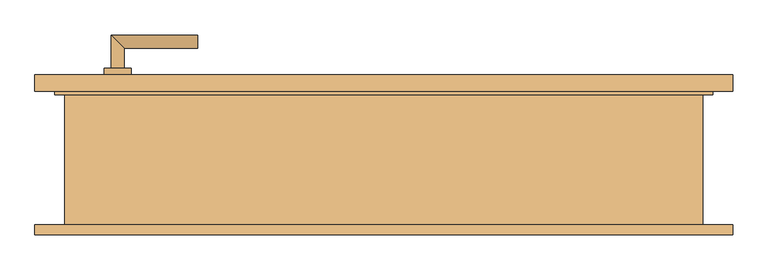
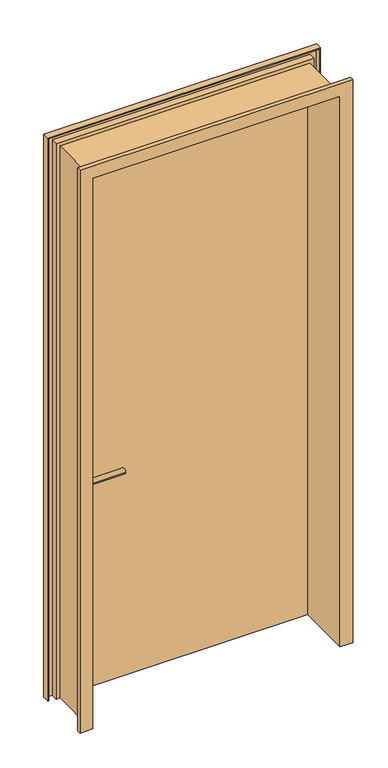
"""IFC4 building model written with IfcOpenShell, lengths in millimetres: door geometry, Drehflügel 1-flg - Variabel : Drehflügel 1-flg - Variabel."""

from ifc_helpers import new_model, si_unit, point, frame, frame_2d, origin, origin_with_axes, place, context, project, spatial, polyline, circle_curve, ellipse_curve, trimmed, segment, composite_curve, outline, extrude, faceted_brep, source, transform, mapped, element, save
from ifc_brep_helpers import plane_surface, cylinder_surface, advanced_brep


def door_75bb7ed5(model_context):
    return source(origin(), model_context, "Body", "SolidModel", [
        advanced_brep(
        [(-410.0, 89.4346141, 900.0), (-390.0, 89.4346141, 900.0), (-410.0, 19.4346141, 900.0), (-390.0, 39.4346141, 900.0), (-280.0, 19.4346141, 900.0), (-280.0, 39.4346141, 900.0)],
        [
            (0, 1, circle_curve(frame((-400.0, 89.4346141, 900.0), z_axis=(0.0, 1.0, 0.0), x_axis=(1.0, 0.0, 0.0)), 10.0)),
            (1, 0, circle_curve(frame((-400.0, 89.4346141, 900.0), z_axis=(0.0, 1.0, 0.0), x_axis=(1.0, 0.0, 0.0)), 10.0)),
            (0, 2),
            (2, 3, ellipse_curve(frame((-400.0, 29.4346141, 900.0), z_axis=(-0.7071067811865385, 0.7071067811865565, 0.0), x_axis=(0.7071067811865563, 0.7071067811865386, 0.0)), 14.1421356, 10.0)),
            (3, 1),
            (3, 2, ellipse_curve(frame((-400.0, 29.4346141, 900.0), z_axis=(-0.7071067811865385, 0.7071067811865565, 0.0), x_axis=(0.7071067811865563, 0.7071067811865386, 0.0)), 14.1421356, 10.0)),
            (4, 5, circle_curve(frame((-280.0, 29.4346141, 900.0), z_axis=(1.0, 0.0, 0.0), x_axis=(0.0, 1.0, 0.0)), 10.0)),
            (5, 4, circle_curve(frame((-280.0, 29.4346141, 900.0), z_axis=(1.0, 0.0, 0.0), x_axis=(0.0, 1.0, 0.0)), 10.0)),
            (2, 4),
            (5, 3),
        ],
        [
            plane_surface(frame((-400.0, 89.4346141, -387.7526403), z_axis=(0.0, 1.0, 0.0), x_axis=(0.0, 0.0, 1.0))),
            cylinder_surface(frame((-400.0, 89.4346141, 900.0), z_axis=(0.0, 1.0, 0.0), x_axis=(1.0, 0.0, 0.0)), 10.0),
            plane_surface(frame((-280.0, 29.4346141, -387.7526403), z_axis=(1.0, 0.0, 0.0), x_axis=(0.0, 0.0, 1.0))),
            cylinder_surface(frame((-400.0, 29.4346141, 900.0), z_axis=(-1.0, 0.0, 0.0), x_axis=(0.0, 1.0, 0.0)), 10.0),
        ],
        [
            (0, [[1, 2]]),
            (1, [[-1, 3, 4, 5]]),
            (1, [[-2, -5, 6, -3]]),
            (2, [[7, 8]]),
            (3, [[-4, 9, -8, 10]]),
            (3, [[-6, -10, -7, -9]]),
        ],
    ),
        advanced_brep(
        [(-390.0, 149.4346141, 900.0), (-410.0, 149.4346141, 900.0), (-390.0, 179.4346141, 900.0), (-410.0, 199.4346141, 900.0), (-280.0, 179.4346141, 900.0), (-280.0, 199.4346141, 900.0)],
        [
            (0, 1, circle_curve(frame((-400.0, 149.4346141, 900.0), z_axis=(0.0, -1.0, 0.0), x_axis=(-1.0, 0.0, 0.0)), 10.0)),
            (1, 0, circle_curve(frame((-400.0, 149.4346141, 900.0), z_axis=(0.0, -1.0, 0.0), x_axis=(-1.0, 0.0, 0.0)), 10.0)),
            (0, 2),
            (2, 3, ellipse_curve(frame((-400.0, 189.4346141, 900.0), z_axis=(-0.7071067811865475, -0.7071067811865475, 0.0), x_axis=(0.7071067811865474, -0.7071067811865476, 0.0)), 14.1421356, 10.0)),
            (3, 1),
            (3, 2, ellipse_curve(frame((-400.0, 189.4346141, 900.0), z_axis=(-0.7071067811865475, -0.7071067811865475, 0.0), x_axis=(0.7071067811865474, -0.7071067811865476, 0.0)), 14.1421356, 10.0)),
            (4, 5, circle_curve(frame((-280.0, 189.4346141, 900.0), z_axis=(1.0, 0.0, 0.0), x_axis=(0.0, 1.0, 0.0)), 10.0)),
            (5, 4, circle_curve(frame((-280.0, 189.4346141, 900.0), z_axis=(1.0, 0.0, 0.0), x_axis=(0.0, 1.0, 0.0)), 10.0)),
            (2, 4),
            (5, 3),
        ],
        [
            plane_surface(frame((-400.0, 149.4346141, -387.7526403), z_axis=(0.0, -1.0, 0.0), x_axis=(0.0, 0.0, 1.0))),
            cylinder_surface(frame((-400.0, 149.4346141, 900.0), z_axis=(0.0, -1.0, 0.0), x_axis=(-1.0, 0.0, 0.0)), 10.0),
            plane_surface(frame((-280.0, 189.4346141, -387.7526403), z_axis=(1.0, 0.0, 0.0), x_axis=(0.0, 0.0, 1.0))),
            cylinder_surface(frame((-400.0, 189.4346141, 900.0), z_axis=(-1.0, 0.0, 0.0), x_axis=(0.0, 1.0, 0.0)), 10.0),
        ],
        [
            (0, [[1, 2]]),
            (1, [[-1, 3, 4, 5]]),
            (1, [[-2, -5, 6, -3]]),
            (2, [[7, 8]]),
            (3, [[-4, 9, -8, 10]]),
            (3, [[-6, -10, -7, -9]]),
        ],
    ),
        extrude(outline(composite_curve([segment(trimmed(circle_curve(frame_2d((900.0, -400.0)), 20.0), [point((900.0, -420.0))], [point((900.0, -380.0))], False, "CARTESIAN"), True, "CONTINUOUS"), segment(trimmed(circle_curve(frame_2d((900.0, -400.0)), 20.0), [point((900.0, -380.0))], [point((900.0, -420.0))], False, "CARTESIAN"), True, "CONTINUOUS")], self_intersect=False)), frame((0.0, 79.4346141, 0.0), z_axis=(0.0, 1.0, 0.0), x_axis=(0.0, 0.0, 1.0)), (0.0, 0.0, 1.0), 10.0),
        extrude(outline(composite_curve([segment(trimmed(circle_curve(frame_2d((900.0, -400.0)), 20.0), [point((900.0, -420.0))], [point((900.0, -380.0))], False, "CARTESIAN"), True, "CONTINUOUS"), segment(trimmed(circle_curve(frame_2d((900.0, -400.0)), 20.0), [point((900.0, -380.0))], [point((900.0, -420.0))], False, "CARTESIAN"), True, "CONTINUOUS")], self_intersect=False)), frame((0.0, 139.4346141, 0.0), z_axis=(0.0, 1.0, 0.0), x_axis=(0.0, 0.0, 1.0)), (0.0, 0.0, 1.0), 10.0),
        extrude(outline(polyline([(490.0, 114.4346141), (-490.0, 114.4346141), (-490.0, 139.4346141), (490.0, 139.4346141), (490.0, 114.4346141)])), origin_with_axes(), (0.0, 0.0, 1.0), 2250.0),
        faceted_brep([(524.4603207, -100.5653859, 0.0), (475.0, -100.5653859, 0.0), (475.0, 114.4346141, 0.0), (490.0, 114.4346141, 0.0), (490.0, 139.4346141, 0.0), (524.4603207, 139.4346141, 0.0), (524.4603207, 114.4346141, 0.0), (519.4603207, 114.4346141, 0.0), (519.4603207, 134.4346141, 0.0), (495.0, 134.4346141, 0.0), (495.0, 109.4346141, 0.0), (480.0, 109.4346141, 0.0), (480.0, -95.5653859, 0.0), (519.4603207, -95.5653859, 0.0), (519.4603207, -85.5653859, 0.0), (524.4603207, -85.5653859, 0.0), (524.4603207, -100.5653859, 2284.4603207), (-524.4603207, -100.5653859, 2284.4603207), (-524.4603207, -100.5653859, 0.0), (-475.0, -100.5653859, 0.0), (-475.0, -100.5653859, 2235.0), (475.0, -100.5653859, 2235.0), (475.0, 114.4346141, 2235.0), (-475.0, 114.4346141, 2235.0), (-475.0, 114.4346141, 0.0), (-490.0, 114.4346141, 0.0), (-490.0, 114.4346141, 2250.0), (490.0, 114.4346141, 2250.0), (490.0, 139.4346141, 2250.0), (-490.0, 139.4346141, 2250.0), (-490.0, 139.4346141, 0.0), (-524.4603207, 139.4346141, 0.0), (-524.4603207, 139.4346141, 2284.4603207), (524.4603207, 139.4346141, 2284.4603207), (524.4603207, 114.4346141, 2284.4603207), (-524.4603207, 114.4346141, 2284.4603207), (-524.4603207, 114.4346141, 0.0), (-519.4603207, 114.4346141, 0.0), (-519.4603207, 114.4346141, 2279.4603207), (519.4603207, 114.4346141, 2279.4603207), (519.4603207, 134.4346141, 2279.4603207), (-519.4603207, 134.4346141, 2279.4603207), (-519.4603207, 134.4346141, 0.0), (-495.0, 134.4346141, 0.0), (-495.0, 134.4346141, 2255.0), (495.0, 134.4346141, 2255.0), (495.0, 109.4346141, 2255.0), (-495.0, 109.4346141, 2255.0), (-495.0, 109.4346141, 0.0), (-480.0, 109.4346141, 0.0), (-480.0, 109.4346141, 2240.0), (480.0, 109.4346141, 2240.0), (480.0, -95.5653859, 2240.0), (-480.0, -95.5653859, 2240.0), (-480.0, -95.5653859, 0.0), (-519.4603207, -95.5653859, 0.0), (-519.4603207, -95.5653859, 2279.4603207), (519.4603207, -95.5653859, 2279.4603207), (519.4603207, -85.5653859, 2279.4603207), (-519.4603207, -85.5653859, 2279.4603207), (-519.4603207, -85.5653859, 0.0), (-524.4603207, -85.5653859, 0.0), (-524.4603207, -85.5653859, 2284.4603207), (524.4603207, -85.5653859, 2284.4603207)], [[[0, 1, 2, 3, 4, 5, 6, 7, 8, 9, 10, 11, 12, 13, 14, 15]], [[1, 0, 16, 17, 18, 19, 20, 21]], [[2, 1, 21, 22]], [[3, 2, 22, 23, 24, 25, 26, 27]], [[4, 3, 27, 28]], [[5, 4, 28, 29, 30, 31, 32, 33]], [[6, 5, 33, 34]], [[7, 6, 34, 35, 36, 37, 38, 39]], [[8, 7, 39, 40]], [[9, 8, 40, 41, 42, 43, 44, 45]], [[10, 9, 45, 46]], [[11, 10, 46, 47, 48, 49, 50, 51]], [[12, 11, 51, 52]], [[13, 12, 52, 53, 54, 55, 56, 57]], [[14, 13, 57, 58]], [[15, 14, 58, 59, 60, 61, 62, 63]], [[0, 15, 63, 16]], [[17, 62, 61, 18]], [[18, 61, 60, 55, 54, 49, 48, 43, 42, 37, 36, 31, 30, 25, 24, 19]], [[23, 20, 19, 24]], [[29, 26, 25, 30]], [[35, 32, 31, 36]], [[41, 38, 37, 42]], [[47, 44, 43, 48]], [[53, 50, 49, 54]], [[59, 56, 55, 60]], [[22, 21, 20, 23]], [[28, 27, 26, 29]], [[34, 33, 32, 35]], [[40, 39, 38, 41]], [[46, 45, 44, 47]], [[52, 51, 50, 53]], [[58, 57, 56, 59]], [[16, 63, 62, 17]]]),
    ])


if __name__ == "__main__":
    model = new_model("IFC4")
    model_context = context("Model", 3, world=origin())
    ifc_project = project(units=[si_unit("LENGTHUNIT", "METRE", prefix="MILLI")], contexts=[model_context])
    site = spatial("IfcSite", under=ifc_project)
    building = spatial("IfcBuilding", under=site)
    placement = place(None, origin())
    door_shape = door_75bb7ed5(model_context)
    element("IfcDoor", 1, ObjectType="Drehflügel 1-flg - Variabel : Drehflügel 1-flg - Variabel", at=placement, inside=building, context=model_context, shape_type="MappedRepresentation", body=[
        mapped(door_shape, transform((0.0, 0.0, 0.0), x_axis=(1.0, 0.0, 0.0), y_axis=(0.0, 1.0, 0.0), z_axis=(0.0, 0.0, 1.0))),
    ])
    save(model, "model.ifc")

# Revit data of these elements
# Type "Drehflügel 1-flg - Variabel : Drehflügel 1-flg - Variabel"
#   Construction Type Id = "MDOOR"
#   Type Mark = "15"
#   Operation = "SingleSwingRight"
#   Keynote = "16.03"
#   Analytic Construction = "Metall"
#   Thermal Resistance (R) = 0.270117 (m²·K)/W
#   Heat Transfer Coefficient (U) = 3.7021 W/(m²·K)
#   Rough Width [instance default] = 1.000 m
#   Rough Height [instance default] = 2.360 m
#   Höhe Türgriff [instance default] = 0.900 m
#   Height [instance default] = 2.260 m
#   Fußbodenaufbau [instance default] = 0.100 m
#   Width [instance default] = 1.000 m
#   Sichtbarkeit Sturzlinien [instance default] = yes
#   Türgriff auswählen [instance default] = element 217699
#   Türgriff [instance default] = none
#   Türflügel [instance default] = none
#   Rahmen/Pfosten [instance default] = Metall - Lackiert - Grau
#   Visual Light Transmittance = 0
#   Solar Heat Gain Coefficient = 0
#   Function = (empty or 0)
#   Wall Closure = (empty or 0)
# Element 1 (IfcDoor, "Drehflügel 1-flg - Variabel : Drehflügel 1-flg - Variabel")
#   Rough Height = 2.260 m
#   Fußbodenaufbau = 0.000 m
#   Materials on its faces: "Metall - Lackiert - Grau", "Metall - Chrom", "Holz - Birke"
# Materials
#   "Metall - Lackiert - Grau": class "Farbe 1", colour RGB 98 98 98, transparency 0, Cost = 0
#   "Metall - Chrom": class "Metall", colour RGB 247 247 247, transparency 0, Cost = 0
#   "Holz - Birke": class "Holz", colour RGB 213 164 103, transparency 0, Cost = 0
